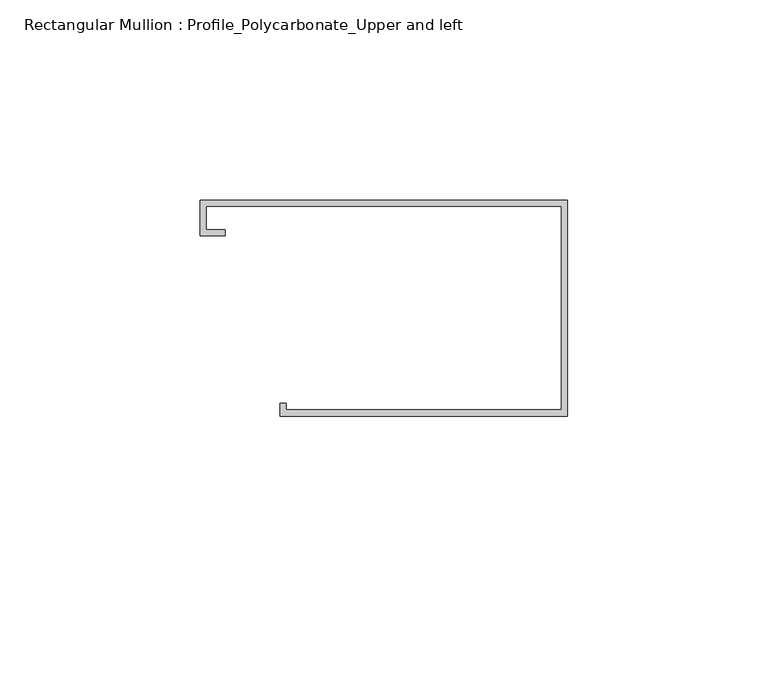
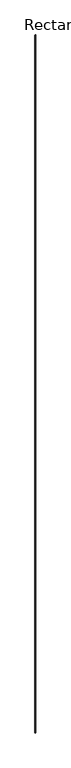
"""IFC4 building model written with IfcOpenShell, lengths in millimetres: member geometry, Rectangular Mullion : Profile_Polycarbonate_Upper and left."""

from ifc_helpers import new_model, si_unit, frame, origin, place, context, project, spatial, polyline, outline, extrude, source, transform, mapped, element, save


def rectangular_mullion_profile_polycarbonate_upper_and_left_b188bb54(model_context):
    return source(origin(), model_context, "Body", "SweptSolid", [
        extrude(outline(polyline([(0.0, 28.984575), (0.0, -25.015825), (-71.9836, -25.015825), (-71.9836, -21.840825), (-70.3961, -21.840825), (-70.3961, -23.428325), (-1.5875, -23.428325), (-1.5875, 27.397075), (-90.4113, 27.397075), (-90.4113, 21.580475), (-85.6488, 21.580475), (-85.6488, 19.992975), (-91.9988, 19.992975), (-91.9988, 28.984575), (0.0, 28.984575)])), frame((0.0, 0.0, -88474.677), z_axis=(0.0, 0.0, 1.0), x_axis=(1.0, 0.0, 0.0)), (0.0, 0.0, 1.0), 88474.677),
    ])


if __name__ == "__main__":
    model = new_model("IFC4")
    model_context = context("Model", 3, world=origin())
    ifc_project = project(units=[si_unit("LENGTHUNIT", "METRE", prefix="MILLI")], contexts=[model_context])
    site = spatial("IfcSite", under=ifc_project)
    building = spatial("IfcBuilding", under=site)
    placement = place(None, origin())
    rectangular_mullion_profile_polycarbonate_upper_and_left_shape = rectangular_mullion_profile_polycarbonate_upper_and_left_b188bb54(model_context)
    element("IfcMember", 1, ObjectType="Rectangular Mullion : Profile_Polycarbonate_Upper and left", at=placement, inside=building, context=model_context, shape_type="MappedRepresentation", body=[
        mapped(rectangular_mullion_profile_polycarbonate_upper_and_left_shape, transform((0.0, 0.0, 0.0), x_axis=(1.0, 0.0, 0.0), y_axis=(0.0, 1.0, 0.0), z_axis=(0.0, 0.0, 1.0))),
    ])
    save(model, "model.ifc")

# Revit data of these elements
# Type "Rectangular Mullion : Profile_Polycarbonate_Upper and left"
#   built-in parameter 1007322 = 0.177167 (stored number, unit not read)
#   built-in parameter 1007321 = 0.00520833 (stored number, unit not read)
#   built-in parameter 1007320 = 0 (stored number, unit not read)
